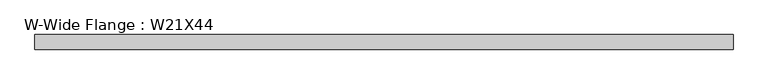
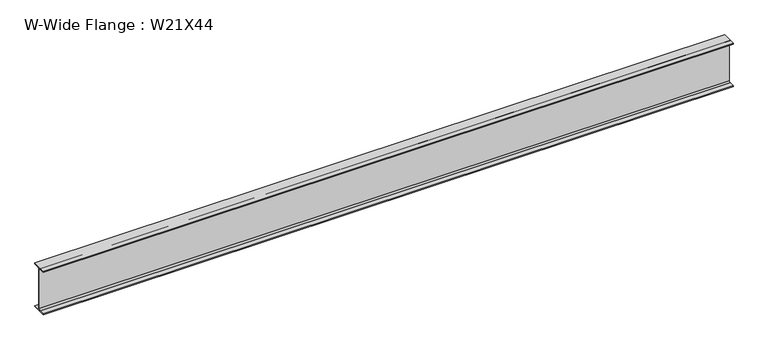
"""IFC4 building model written with IfcOpenShell, lengths in millimetres: beam geometry, W-Wide Flange : W21X44."""

from ifc_helpers import new_model, si_unit, point, frame, frame_2d, origin, place, context, project, spatial, polyline, circle_curve, trimmed, segment, composite_curve, outline, extrude, source, transform, mapped, element, save


def w_wide_flange_w21x44_42aa095b(model_context):
    return source(origin(), model_context, "Body", "SweptSolid", [
        extrude(outline(composite_curve([segment(polyline([(82.55, -251.46), (82.55, -262.89), (-82.55, -262.89), (-82.55, -251.46), (-21.59, -251.46)]), True, "CONTINUOUS"), segment(trimmed(circle_curve(frame_2d((-21.59, -234.315)), 17.145), [point((-21.59, -251.46))], [point((-4.445, -234.315))], True, "CARTESIAN"), True, "CONTINUOUS"), segment(polyline([(-4.445, -234.315), (-4.445, 234.315)]), True, "CONTINUOUS"), segment(trimmed(circle_curve(frame_2d((-21.59, 234.315)), 17.145), [point((-4.445, 234.315))], [point((-21.59, 251.46))], True, "CARTESIAN"), True, "CONTINUOUS"), segment(polyline([(-21.59, 251.46), (-82.55, 251.46), (-82.55, 262.89), (82.55, 262.89), (82.55, 251.46), (21.59, 251.46)]), True, "CONTINUOUS"), segment(trimmed(circle_curve(frame_2d((21.59, 234.315)), 17.145), [point((21.59, 251.46))], [point((4.445, 234.315))], True, "CARTESIAN"), True, "CONTINUOUS"), segment(polyline([(4.445, 234.315), (4.445, -234.315)]), True, "CONTINUOUS"), segment(trimmed(circle_curve(frame_2d((21.59, -234.315)), 17.145), [point((4.445, -234.315))], [point((21.59, -251.46))], True, "CARTESIAN"), True, "CONTINUOUS"), segment(polyline([(21.59, -251.46), (82.55, -251.46)]), True, "CONTINUOUS")], self_intersect=False)), frame((-3902.8387461, 0.0, 0.0), z_axis=(1.0, 0.0, 0.0), x_axis=(0.0, 1.0, 0.0)), (0.0, 0.0, 1.0), 7866.3808046),
    ])


if __name__ == "__main__":
    model = new_model("IFC4")
    model_context = context("Model", 3, world=origin())
    ifc_project = project(units=[si_unit("LENGTHUNIT", "METRE", prefix="MILLI")], contexts=[model_context])
    site = spatial("IfcSite", under=ifc_project)
    building = spatial("IfcBuilding", under=site)
    placement = place(None, origin())
    w_wide_flange_w21x44_shape = w_wide_flange_w21x44_42aa095b(model_context)
    element("IfcBeam", 1, ObjectType="W-Wide Flange : W21X44", at=placement, inside=building, context=model_context, shape_type="MappedRepresentation", body=[
        mapped(w_wide_flange_w21x44_shape, transform((0.0, 0.0, 0.0), x_axis=(1.0, 0.0, 0.0), y_axis=(0.0, 1.0, 0.0), z_axis=(0.0, 0.0, 1.0))),
    ])
    save(model, "model.ifc")

# Revit data of these elements
# Type "W-Wide Flange : W21X44"
#   Assembly Code = "B10"
#   W = 44
#   Length [instance default] = 1524 mm
#   bf = 165.1 mm
#   d = 525.78 mm
#   k = 28.575 mm
#   k2 = 17.145 mm
#   tf = 11.43 mm
#   tw = 8.89 mm
#   A = 0.00838708 m²
#   Structural Material [instance default] = Steel ASTM A992
# Element 1 (IfcBeam, "W-Wide Flange : W21X44")
#   Structural Material = Aluminum, Anodized Red
#   Materials on its faces: "Aluminum, Anodized Red"
# Materials
#   "Steel ASTM A992": class "Metal", colour RGB 128 0 0, transparency 0, Description = "Structural steel 50ksi", Cost = 0
#   "Aluminum, Anodized Red": class "Metal", colour RGB 120 120 120, transparency 0, Description = "Anodized aluminum, red", Cost = 0
